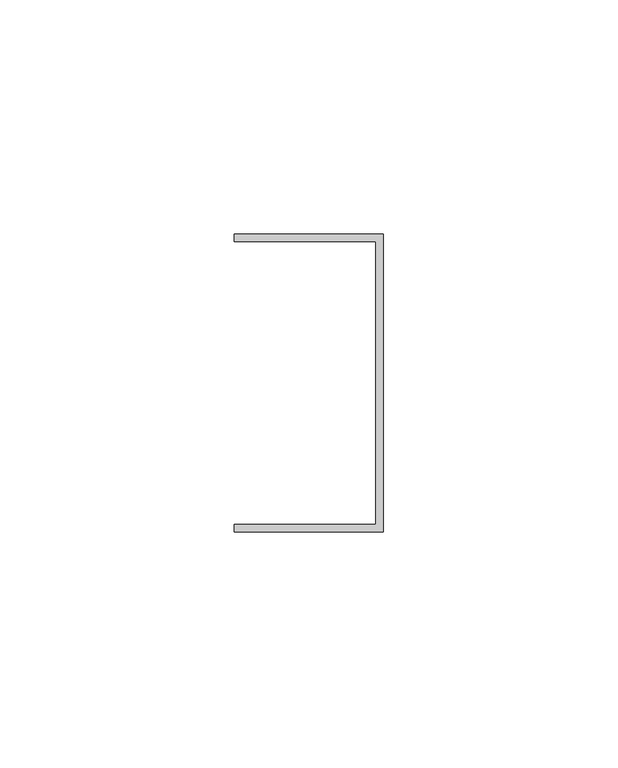
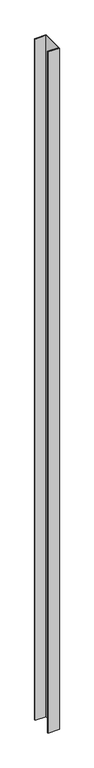
"""IFC4 building model written with IfcOpenShell, lengths in millimetres: proxy geometry, Generic Models 7:Generic Models 1:3:Generic Models 1:3 : Generic Models 7:Generic Models 1:305549:3:Generic Models 1:3:Generic Models 1:3 : Generic Models 7:Generic Models 1:305549:3 : Generic Models 7:Generic Models 1:3:Generic Models 1:3 : Generic Models 7:Generic Models 1:305549:301244:10 : Generic Models 7:Generic Models 1:3:Generic Models 1:3 : Generic Models 7:Generic Models 1:305549:3:Generic Models 1:3:Generic Models 1:3 : Generic Models 7:Generic Models 1:305549:3 : Generic Models 7:Generic Models 1:3:Generic Models 1:3 : Generic Models 7:Generic Models 1:305549:301244:308848."""

from ifc_helpers import new_model, si_unit, frame, origin, place, context, project, spatial, polyline, outline, extrude, source, transform, mapped, element, save


def generic_models_e0e0a2f4(model_context):
    return source(origin(), model_context, "Body", "SweptSolid", [
        extrude(outline(polyline([(579307.7117239, -579013.3913842), (579307.7117239, -579076.891384), (579275.9617239, -579076.891384), (579275.9617239, -579075.303884), (579306.1242239, -579075.303884), (579306.1242239, -579014.9788842), (579275.9617239, -579014.9788842), (579275.9617239, -579013.3913842), (579307.7117239, -579013.3913842)])), frame((0.0, 0.0, 4133.81326), z_axis=(0.0, 0.0, 1.0), x_axis=(1.0, 0.0, 0.0)), (0.0, 0.0, 1.0), 2000.28674),
    ])


if __name__ == "__main__":
    model = new_model("IFC4")
    model_context = context("Model", 3, world=origin())
    ifc_project = project(units=[si_unit("LENGTHUNIT", "METRE", prefix="MILLI")], contexts=[model_context])
    site = spatial("IfcSite", under=ifc_project)
    building = spatial("IfcBuilding", under=site)
    placement = place(None, origin())
    generic_models_shape = generic_models_e0e0a2f4(model_context)
    element("IfcBuildingElementProxy", 1, Name="Generic Models 7:Generic Models 1:3:Generic Models 1:3 : Generic Models 7:Generic Models 1:305549:3:Generic Models 1:3:Generic Models 1:3 : Generic Models 7:Generic Models 1:305549:3 : Generic Models 7:Generic Models 1:3:Generic Models 1:3 : Generic Models 7:Generic Models 1:305549:301244:10 : Generic Models 7:Generic Models 1:3:Generic Models 1:3 : Generic Models 7:Generic Models 1:305549:3:Generic Models 1:3:Generic Models 1:3 : Generic Models 7:Generic Models 1:305549:3 : Generic Models 7:Generic Models 1:3:Generic Models 1:3 : Generic Models 7:Generic Models 1:305549:301244:308848", ObjectType="Generic Models 7:Generic Models 1:3:Generic Models 1:3 : Generic Models 7:Generic Models 1:305549:3:Generic Models 1:3:Generic Models 1:3 : Generic Models 7:Generic Models 1:305549:3 : Generic Models 7:Generic Models 1:3:Generic Models 1:3 : Generic Models 7:Generic Models 1:305549:301244:10 : Generic Models 7:Generic Models 1:3:Generic Models 1:3 : Generic Models 7:Generic Models 1:305549:3:Generic Models 1:3:Generic Models 1:3 : Generic Models 7:Generic Models 1:305549:3 : Generic Models 7:Generic Models 1:3:Generic Models 1:3 : Generic Models 7:Generic Models 1:305549:301244:308848", at=placement, inside=building, context=model_context, shape_type="MappedRepresentation", body=[
        mapped(generic_models_shape, transform((0.0, 0.0, 0.0), x_axis=(1.0, 0.0, 0.0), y_axis=(0.0, 1.0, 0.0), z_axis=(0.0, 0.0, 1.0))),
    ])
    save(model, "model.ifc")

# Revit data of these elements
# Type "Generic Models 7:Generic Models 1:3:Generic Models 1:3 : Generic Models 7:Generic Models 1:305549:3:Generic Models 1:3:Generic Models 1:3 : Generic Models 7:Generic Models 1:305549:3 : Generic Models 7:Generic Models 1:3:Generic Models 1:3 : Generic Models 7:Generic Models 1:305549:301244:10 : Generic Models 7:Generic Models 1:3:Generic Models 1:3 : Generic Models 7:Generic Models 1:305549:3:Generic Models 1:3:Generic Models 1:3 : Generic Models 7:Generic Models 1:305549:3 : Generic Models 7:Generic Models 1:3:Generic Models 1:3 : Generic Models 7:Generic Models 1:305549:301244:308848"
#   NameOverride = "Generic Models 7:Generic Models 1:3:Generic Models 1:3 : Generic Models 7:Generic Models 1:305549:3:Generic Models 1:3:Generic Models 1:3 : Generic Models 7:Generic Models 1:305549:3 : Generic Models 7:Generic Models 1:3:Generic Models 1:3 : Generic Models 7:Generic Models 1:305549:301244:308848"
#   ObjectTypeOverride = "Generic Models 1:3:Generic Models 1:3 : Generic Models 7:Generic Models 1:305549:3 : Generic Models 7:Generic Models 1:3:Generic Models 1:3 : Generic Models 7:Generic Models 1:305549:301244"
#   Reference = "Generic Models 1"
#   Tag = "308848"
# Element 1 (IfcBuildingElementProxy, "Generic Models 7:Generic Models 1:3:Generic Models 1:3 : Generic Models 7:Generic Models 1:305549:3:Generic Models 1:3:Generic Models 1:3 : Generic Models 7:Generic Models 1:305549:3 : Generic Models 7:Generic Models 1:3:Generic Models 1:3 : Generic Models 7:Generic Models 1:305549:301244:10 : Generic Models 7:Generic Models 1:3:Generic Models 1:3 : Generic Models 7:Generic Models 1:305549:3:Generic Models 1:3:Generic Models 1:3 : Generic Models 7:Generic Models 1:305549:3 : Generic Models 7:Generic Models 1:3:Generic Models 1:3 : Generic Models 7:Generic Models 1:305549:301244:308848")
#   Materials on its faces: "GALVANIZED U-CHANNEL (250T125-33)"
# Materials
#   "GALVANIZED U-CHANNEL (250T125-33)": class "Unassigned", colour RGB 202 201 200, transparency 0, Keynote = "M05451300.02", Cost = 0
